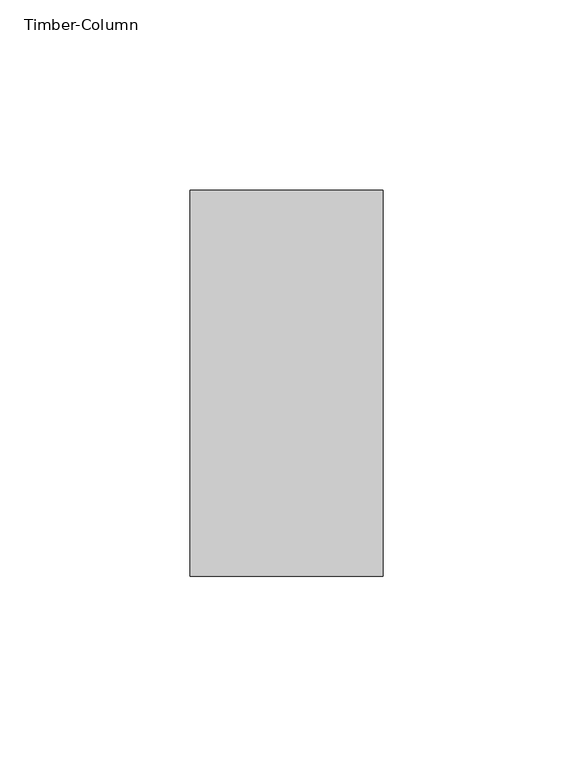
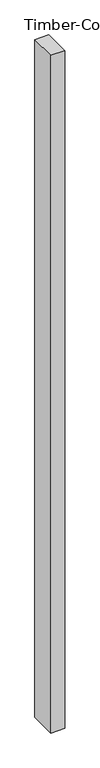
"""IFC4 building model written with IfcOpenShell, lengths in millimetres: column geometry, Timber-Column."""

from ifc_helpers import new_model, si_unit, frame, origin, place, context, project, spatial, polyline, outline, extrude, source, transform, mapped, element, save


def timber_column_65e54e3c(model_context):
    return source(origin(), model_context, "Body", "SweptSolid", [
        extrude(outline(polyline([(25.4, 50.8), (25.4, -50.8), (-25.4, -50.8), (-25.4, 50.8), (25.4, 50.8)])), frame((0.0, 0.0, 50.8), z_axis=(0.0, 0.0, 1.0), x_axis=(1.0, 0.0, 0.0)), (0.0, 0.0, 1.0), 2616.2),
    ])


if __name__ == "__main__":
    model = new_model("IFC4")
    model_context = context("Model", 3, world=origin())
    ifc_project = project(units=[si_unit("LENGTHUNIT", "METRE", prefix="MILLI")], contexts=[model_context])
    site = spatial("IfcSite", under=ifc_project)
    building = spatial("IfcBuilding", under=site)
    placement = place(None, origin())
    timber_column_shape = timber_column_65e54e3c(model_context)
    element("IfcColumn", 1, ObjectType="Timber-Column : BLDG 6241 Wall Struds 2\"x4\"", at=placement, inside=building, context=model_context, shape_type="MappedRepresentation", body=[
        mapped(timber_column_shape, transform((0.0, 0.0, 0.0), x_axis=(1.0, 0.0, 0.0), y_axis=(0.0, 1.0, 0.0), z_axis=(0.0, 0.0, 1.0))),
    ])
    save(model, "model.ifc")

# Revit data of these elements
# Type "Timber-Column : BLDG 6241 Wall Struds 2\"x4\""
#   Assembly Code = "B10"
#   A = 0.140625 SF
#   b = 0' - 2"
#   d = 0' - 4"
#   Structural Material [instance default] = Softwood, Lumber
# Element 1 (IfcColumn, "Timber-Column : BLDG 6241 Wall Struds 2\"x4\"")
#   Materials on its faces: "Softwood, Lumber"
# Materials
#   "Softwood, Lumber": class "Wood", colour RGB 223 192 134, transparency 0, Description = "Pinus Echinata", Cost = 0
